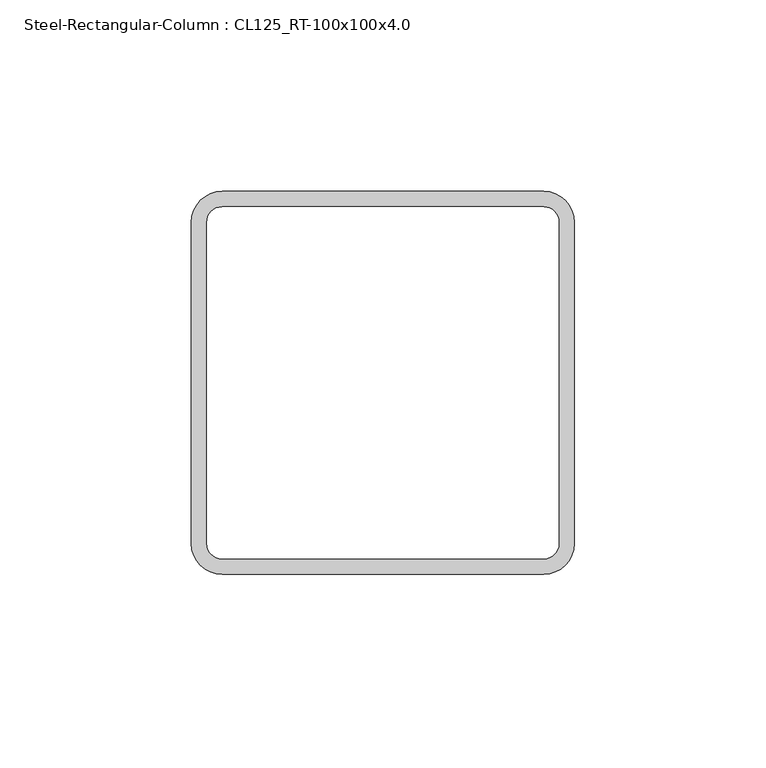
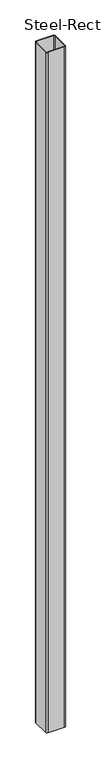
"""IFC4 building model written with IfcOpenShell, lengths in millimetres: column geometry, Steel-Rectangular-Column : CL125_RT-100x100x4.0."""

from ifc_helpers import new_model, si_unit, point, frame, frame_2d, origin, place, context, project, spatial, polyline, circle_curve, trimmed, segment, composite_curve, outline, extrude, source, transform, mapped, element, save


def steel_rectangular_column_cl125_rt_100x100x4_0_3623087c(model_context):
    return source(origin(), model_context, "Body", "SweptSolid", [
        extrude(outline(composite_curve([segment(polyline([(42.0, -50.0), (-42.0, -50.0)]), True, "CONTINUOUS"), segment(trimmed(circle_curve(frame_2d((-42.0, -42.0)), 8.0), [point((-42.0, -50.0))], [point((-50.0, -42.0))], False, "CARTESIAN"), True, "CONTINUOUS"), segment(polyline([(-50.0, -42.0), (-50.0, 42.0)]), True, "CONTINUOUS"), segment(trimmed(circle_curve(frame_2d((-42.0, 42.0)), 8.0), [point((-50.0, 42.0))], [point((-42.0, 50.0))], False, "CARTESIAN"), True, "CONTINUOUS"), segment(polyline([(-42.0, 50.0), (42.0, 50.0)]), True, "CONTINUOUS"), segment(trimmed(circle_curve(frame_2d((42.0, 42.0)), 8.0), [point((42.0, 50.0))], [point((50.0, 42.0))], False, "CARTESIAN"), True, "CONTINUOUS"), segment(polyline([(50.0, 42.0), (50.0, -42.0)]), True, "CONTINUOUS"), segment(trimmed(circle_curve(frame_2d((42.0, -42.0)), 8.0), [point((50.0, -42.0))], [point((42.0, -50.0))], False, "CARTESIAN"), True, "CONTINUOUS")], self_intersect=False), holes=[composite_curve([segment(trimmed(circle_curve(frame_2d((42.0, -42.0)), 4.0), [point((42.0, -46.0))], [point((46.0, -42.0))], True, "CARTESIAN"), True, "CONTINUOUS"), segment(polyline([(46.0, -42.0), (46.0, 42.0)]), True, "CONTINUOUS"), segment(trimmed(circle_curve(frame_2d((42.0, 42.0)), 4.0), [point((46.0, 42.0))], [point((42.0, 46.0))], True, "CARTESIAN"), True, "CONTINUOUS"), segment(polyline([(42.0, 46.0), (-42.0, 46.0)]), True, "CONTINUOUS"), segment(trimmed(circle_curve(frame_2d((-42.0, 42.0)), 4.0), [point((-42.0, 46.0))], [point((-46.0, 42.0))], True, "CARTESIAN"), True, "CONTINUOUS"), segment(polyline([(-46.0, 42.0), (-46.0, -42.0)]), True, "CONTINUOUS"), segment(trimmed(circle_curve(frame_2d((-42.0, -42.0)), 4.0), [point((-46.0, -42.0))], [point((-42.0, -46.0))], True, "CARTESIAN"), True, "CONTINUOUS"), segment(polyline([(-42.0, -46.0), (42.0, -46.0)]), True, "CONTINUOUS")], self_intersect=False)]), frame((0.0, 0.0, 1400.0), z_axis=(0.0, 0.0, 1.0), x_axis=(1.0, 0.0, 0.0)), (0.0, 0.0, 1.0), 3600.0),
    ])


if __name__ == "__main__":
    model = new_model("IFC4")
    model_context = context("Model", 3, world=origin())
    ifc_project = project(units=[si_unit("LENGTHUNIT", "METRE", prefix="MILLI")], contexts=[model_context])
    site = spatial("IfcSite", under=ifc_project)
    building = spatial("IfcBuilding", under=site)
    placement = place(None, origin())
    steel_rectangular_column_cl125_rt_100x100x4_0_shape = steel_rectangular_column_cl125_rt_100x100x4_0_3623087c(model_context)
    element("IfcColumn", 1, ObjectType="Steel-Rectangular-Column : CL125_RT-100x100x4.0", at=placement, inside=building, context=model_context, shape_type="MappedRepresentation", body=[
        mapped(steel_rectangular_column_cl125_rt_100x100x4_0_shape, transform((0.0, 0.0, 0.0), x_axis=(1.0, 0.0, 0.0), y_axis=(0.0, 1.0, 0.0), z_axis=(0.0, 0.0, 1.0))),
    ])
    save(model, "model.ifc")

# Revit data of these elements
# Type "Steel-Rectangular-Column : CL125_RT-100x100x4.0"
#   Surface Area = 0.386 m²/m
#   b = 100 mm
#   h = 100 mm
#   tr = 8 mm
#   t = 4 mm
#   Section Area = 14.95 cm²
#   Mass per Unit Length = 11.70 kg/m
#   hec_material4 [instance default] = none
#   hec_material3 [instance default] = none
#   hec_material2 [instance default] = none
#   hec_material1 [instance default] = none
#   Structural Material [instance default] = Steel, 45-345
# Element 1 (IfcColumn, "Steel-Rectangular-Column : CL125_RT-100x100x4.0")
#   Structural Material = S01AA007-00001_Main Steel Structure Fabrication Work_Shelter/Building_Girth & Purlin
#   Materials on its faces: "S01AA007-00001_Main Steel Structure Fabrication Work_Shelter/Building_Girth & Purlin"
# Materials
#   "Steel, 45-345": class "Metal", colour RGB 189 187 185, transparency 0, Description = "Steel 345 MPa", Cost = 0
#   "S01AA007-00001_Main Steel Structure Fabrication Work_Shelter/Building_Girth & Purlin": class "Metal", colour RGB 120 120 120, transparency 0, Comments = "(30KG/M>Weight)", Description = "Structural steel 50ksi", W00) Work Master Code = "S01AA007-00001", W01) Work Master_Lv1 = "Main Steel Structure Fabrication Work", W02) Work Master_Lv2 = "Shelter/Building", W03) Work Master_Spec.1 = "Girth & Purlin", Cost = 0
